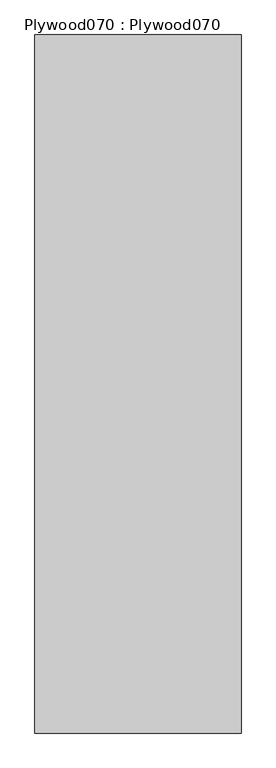
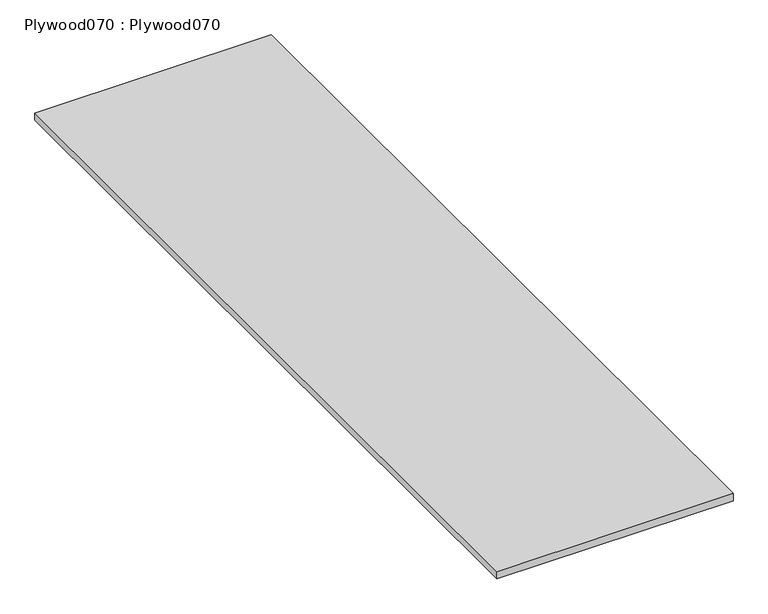
"""IFC4 building model written with IfcOpenShell, lengths in millimetres: proxy geometry, Plywood070 : Plywood070."""

from ifc_helpers import new_model, si_unit, frame, origin, place, context, project, spatial, polyline, outline, extrude, source, transform, mapped, element, save


def plywood070_plywood070_da915f52(model_context):
    return source(origin(), model_context, "Body", "SweptSolid", [
        extrude(outline(polyline([(-6632.5776325, 7982.1531721), (-7223.1276325, 7982.1531721), (-7223.1276325, 9982.1531721), (-6632.5776325, 9982.1531721), (-6632.5776325, 7982.1531721)])), frame((0.0, 0.0, 39560.2460083), z_axis=(0.0, 0.0, 1.0), x_axis=(1.0, 0.0, 0.0)), (0.0, 0.0, 1.0), 19.05),
    ])


if __name__ == "__main__":
    model = new_model("IFC4")
    model_context = context("Model", 3, world=origin())
    ifc_project = project(units=[si_unit("LENGTHUNIT", "METRE", prefix="MILLI")], contexts=[model_context])
    site = spatial("IfcSite", under=ifc_project)
    building = spatial("IfcBuilding", under=site)
    placement = place(None, origin())
    plywood070_plywood070_shape = plywood070_plywood070_da915f52(model_context)
    element("IfcBuildingElementProxy", 1, Name="Plywood070 : Plywood070", ObjectType="Plywood070 : Plywood070", at=placement, inside=building, context=model_context, shape_type="MappedRepresentation", body=[
        mapped(plywood070_plywood070_shape, transform((0.0, 0.0, 0.0), x_axis=(1.0, 0.0, 0.0), y_axis=(0.0, 1.0, 0.0), z_axis=(0.0, 0.0, 1.0))),
    ])
    save(model, "model.ifc")

# Revit data of these elements
# Type "Plywood070 : Plywood070"
#   NameOverride = "Plywood070"
# Element 1 (IfcBuildingElementProxy, "Plywood070 : Plywood070")
#   Materials on its faces: "CDX PLYWOOD -  SEE STRUCTURAL DWGS"
# Materials
#   "CDX PLYWOOD -  SEE STRUCTURAL DWGS": class "Unassigned", colour RGB 177 130 114, transparency 0, Cost = 0
